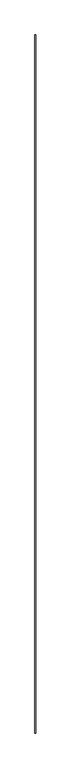
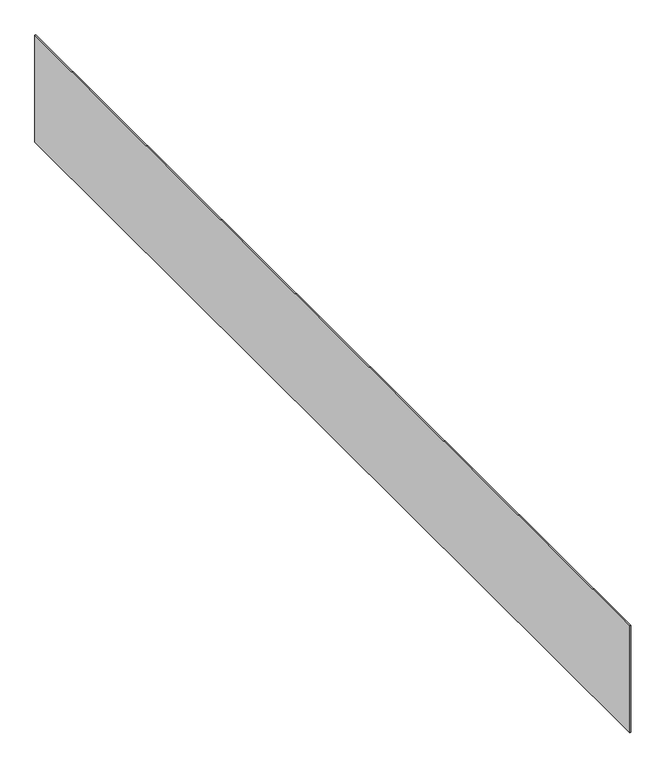
"""IFC4 building model written with IfcOpenShell, lengths in millimetres: proxy geometry, Generic Models 7:Generic Models 1:5:Generic Models 1:5 : Generic Models 7:Generic Models 1:337419:29 : Generic Models 7:Generic Models 1:5:Generic Models 1:5 : Generic Models 7:Generic Models 1:337419:311462."""

from ifc_helpers import new_model, si_unit, frame, origin, place, context, project, spatial, polyline, outline, extrude, source, transform, mapped, element, save


def generic_models_df8c19f0(model_context):
    return source(origin(), model_context, "Body", "SweptSolid", [
        extrude(outline(polyline([(579326.7617241, -560020.541384), (579345.8117241, -560020.541384), (579345.8117239, -579008.999326), (579326.7617239, -579008.999326), (579326.7617241, -560020.541384)])), frame((0.0, 0.0, 4073.3832563), z_axis=(0.0, 0.0, 1.0), x_axis=(1.0, 0.0, 0.0)), (0.0, 0.0, 1.0), 2081.7076927),
    ])


if __name__ == "__main__":
    model = new_model("IFC4")
    model_context = context("Model", 3, world=origin())
    ifc_project = project(units=[si_unit("LENGTHUNIT", "METRE", prefix="MILLI")], contexts=[model_context])
    site = spatial("IfcSite", under=ifc_project)
    building = spatial("IfcBuilding", under=site)
    placement = place(None, origin())
    generic_models_shape = generic_models_df8c19f0(model_context)
    element("IfcBuildingElementProxy", 1, Name="Generic Models 7:Generic Models 1:5:Generic Models 1:5 : Generic Models 7:Generic Models 1:337419:29 : Generic Models 7:Generic Models 1:5:Generic Models 1:5 : Generic Models 7:Generic Models 1:337419:311462", ObjectType="Generic Models 7:Generic Models 1:5:Generic Models 1:5 : Generic Models 7:Generic Models 1:337419:29 : Generic Models 7:Generic Models 1:5:Generic Models 1:5 : Generic Models 7:Generic Models 1:337419:311462", at=placement, inside=building, context=model_context, shape_type="MappedRepresentation", body=[
        mapped(generic_models_shape, transform((0.0, 0.0, 0.0), x_axis=(1.0, 0.0, 0.0), y_axis=(0.0, 1.0, 0.0), z_axis=(0.0, 0.0, 1.0))),
    ])
    save(model, "model.ifc")

# Revit data of these elements
# Type "Generic Models 7:Generic Models 1:5:Generic Models 1:5 : Generic Models 7:Generic Models 1:337419:29 : Generic Models 7:Generic Models 1:5:Generic Models 1:5 : Generic Models 7:Generic Models 1:337419:311462"
#   NameOverride = "Generic Models 7:Generic Models 1:5:Generic Models 1:5 : Generic Models 7:Generic Models 1:337419:311462"
#   ObjectTypeOverride = "Generic Models 1:5 : Generic Models 7:Generic Models 1:337419"
#   Reference = "Generic Models 1"
#   Tag = "311462"
# Element 1 (IfcBuildingElementProxy, "Generic Models 7:Generic Models 1:5:Generic Models 1:5 : Generic Models 7:Generic Models 1:337419:29 : Generic Models 7:Generic Models 1:5:Generic Models 1:5 : Generic Models 7:Generic Models 1:337419:311462")
#   Materials on its faces: "1\" MINERAL WOOL BOARD INSULATION - BLACK MAT FACER"
# Materials
#   "1\" MINERAL WOOL BOARD INSULATION - BLACK MAT FACER": class "Unassigned", colour RGB 205 188 106, transparency 0, Cost = 0
